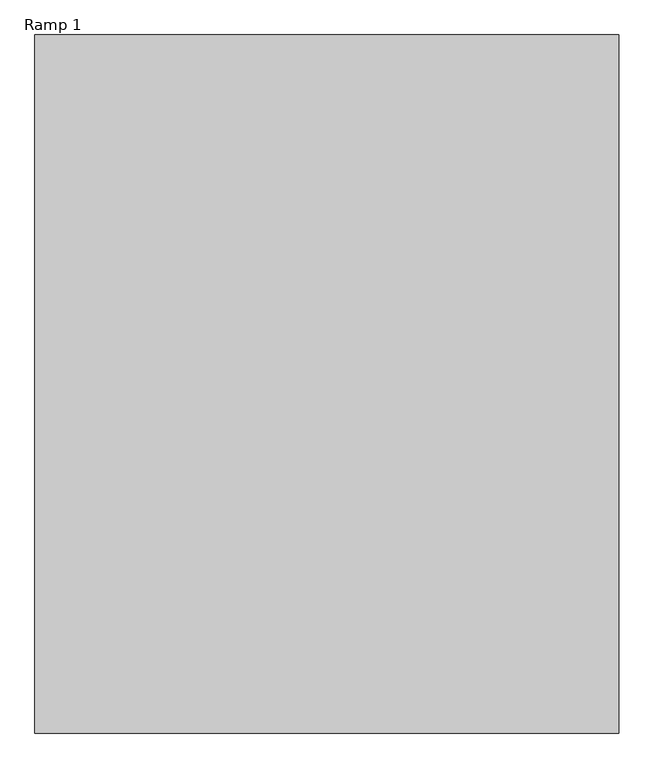
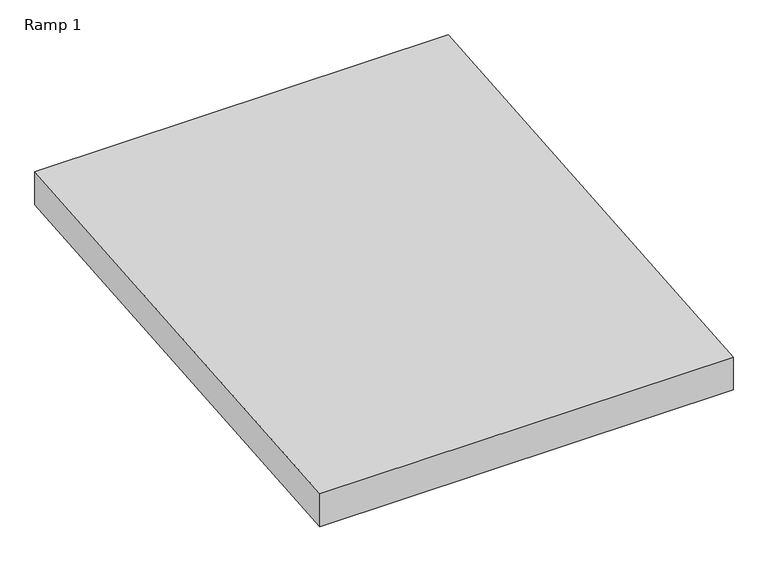
"""IFC4 building model written with IfcOpenShell, lengths in millimetres: ramp geometry, Ramp 1."""

import ifcopenshell
import ifcopenshell.guid

model = None  # the IFC model being written
_history = None  # IfcOwnerHistory: only IFC2X3 demands one
_inside = {}  # id of a spatial element -> (the spatial element, [elements in it])
_under = {}  # id of a project, library or spatial element -> (it, [spatial elements below it])
_declared = {}  # id of a project -> (the project, [libraries it declares])
_typed = {}  # id of a type object -> (the type object, [elements of that type])
_made_of = {}  # id of a material, layer set ... -> (it, [elements and type objects made of it])


def new_model(schema):
    """Start an empty IFC model of exactly this schema.

    Asked for "IFC4X3", IfcOpenShell would pick the latest addendum, in which some entities
    have other attributes; the version numbers below select the first issue.
    IFC2X3 requires an IfcOwnerHistory on every rooted entity: one is made here for all.
    """
    global model, _history
    if schema == "IFC4X3":
        model = ifcopenshell.file(schema_version=(4, 3, 0, 0))
    else:
        model = ifcopenshell.file(schema=schema)
    _inside.clear()
    _under.clear()
    _declared.clear()
    _typed.clear()
    _made_of.clear()
    _history = None
    if model.schema == "IFC2X3":
        org = make("IfcOrganization", Name="unknown")
        user = make(
            "IfcPersonAndOrganization",
            ThePerson=make("IfcPerson", FamilyName="unknown"),
            TheOrganization=org,
        )
        app = make(
            "IfcApplication",
            ApplicationDeveloper=org,
            Version="unknown",
            ApplicationFullName="unknown",
            ApplicationIdentifier="unknown",
        )
        _history = make(
            "IfcOwnerHistory",
            OwningUser=user,
            OwningApplication=app,
            ChangeAction="ADDED",
            CreationDate=0,
        )
    return model


def make(cls, **values):
    """One entity of the class cls with the attributes given. An attribute that is None is left unset."""
    return model.create_entity(
        cls, **{name: value for name, value in values.items() if value is not None}
    )


def rooted(cls, **values):
    """An entity with a GlobalId (a new one), such as an element, a storey or a relation."""
    return make(cls, GlobalId=ifcopenshell.guid.new(), OwnerHistory=_history, **values)


def si_unit(unit_type, name, prefix=None):
    """IfcSIUnit, for example si_unit("LENGTHUNIT", "METRE", prefix="MILLI")."""
    return make("IfcSIUnit", UnitType=unit_type, Prefix=prefix, Name=name)


def assignment(units):
    """IfcUnitAssignment: the units of a project."""
    return None if units is None else make("IfcUnitAssignment", Units=units)


def point(xyz):
    """IfcCartesianPoint."""
    return None if xyz is None else make("IfcCartesianPoint", Coordinates=xyz)


def direction(xyz):
    """IfcDirection."""
    return None if xyz is None else make("IfcDirection", DirectionRatios=xyz)


def frame(location, z_axis=None, x_axis=None):
    """IfcAxis2Placement3D, a coordinate frame: its origin and axes. An axis left out is left unset."""
    return make(
        "IfcAxis2Placement3D",
        Location=point(location),
        Axis=direction(z_axis),
        RefDirection=direction(x_axis),
    )


def origin():
    """The frame at (0, 0, 0) with its axes left unset."""
    return frame((0.0, 0.0, 0.0))


def place(relative_to, where):
    """IfcLocalPlacement: puts the frame where relative to a parent placement (None: the world)."""
    return make(
        "IfcLocalPlacement", PlacementRelTo=relative_to, RelativePlacement=where
    )


def context(
    kind, dimensions, precision=None, world=None, true_north=None, identifier=None
):
    """IfcGeometricRepresentationContext, for example the 3D "Model" context."""
    return make(
        "IfcGeometricRepresentationContext",
        ContextIdentifier=identifier,
        ContextType=kind,
        CoordinateSpaceDimension=dimensions,
        Precision=precision,
        WorldCoordinateSystem=world,
        TrueNorth=true_north,
    )


def project(units=None, contexts=None):
    """IfcProject with its units and contexts."""
    return rooted(
        "IfcProject",
        Name="project",
        RepresentationContexts=contexts,
        UnitsInContext=assignment(units),
    )


def spatial(cls, under=None, at=None, **own):
    """A site, building, storey or space (cls), placed at a placement, below another one or the project."""
    s = rooted(cls, ObjectPlacement=at, **own)
    if under is not None:
        _under.setdefault(under.id(), (under, []))[1].append(s)
    return s


def polyline(points):
    """IfcPolyline through the points."""
    return make("IfcPolyline", Points=[point(p) for p in points])


def outline(outer, holes=None, kind="AREA"):
    """IfcArbitraryClosedProfileDef: a profile drawn as a closed curve; with holes, ...WithVoids."""
    if holes is None:
        return make("IfcArbitraryClosedProfileDef", ProfileType=kind, OuterCurve=outer)
    return make(
        "IfcArbitraryProfileDefWithVoids",
        ProfileType=kind,
        OuterCurve=outer,
        InnerCurves=holes,
    )


def extrude(swept, where, along, depth):
    """IfcExtrudedAreaSolid: the profile swept, set in the frame where, extruded along a direction by depth."""
    return make(
        "IfcExtrudedAreaSolid",
        SweptArea=swept,
        Position=where,
        ExtrudedDirection=direction(along),
        Depth=depth,
    )


def shape(context_of_items, identifier, shape_type, items):
    """IfcShapeRepresentation: the items that make up one representation, for example the "Body"."""
    return make(
        "IfcShapeRepresentation",
        ContextOfItems=context_of_items,
        RepresentationIdentifier=identifier,
        RepresentationType=shape_type,
        Items=items,
    )


def source(mapping_origin, context_of_items, identifier, shape_type, items):
    """IfcRepresentationMap: a shape defined once, which mapped items show again and again."""
    return make(
        "IfcRepresentationMap",
        MappingOrigin=mapping_origin,
        MappedRepresentation=shape(context_of_items, identifier, shape_type, items),
    )


def transform(
    local_origin,
    x_axis=None,
    y_axis=None,
    z_axis=None,
    scale=None,
    scale2=None,
    scale3=None,
    uniform=True,
):
    """IfcCartesianTransformationOperator3D, or its non-uniform kind. x_axis, y_axis, z_axis: its Axis1, 2, 3."""
    if uniform:
        return make(
            "IfcCartesianTransformationOperator3D",
            Axis1=direction(x_axis),
            Axis2=direction(y_axis),
            LocalOrigin=point(local_origin),
            Scale=scale,
            Axis3=direction(z_axis),
        )
    return make(
        "IfcCartesianTransformationOperator3DnonUniform",
        Axis1=direction(x_axis),
        Axis2=direction(y_axis),
        LocalOrigin=point(local_origin),
        Scale=scale,
        Axis3=direction(z_axis),
        Scale2=scale2,
        Scale3=scale3,
    )


def mapped(mapping_source, mapping_target):
    """IfcMappedItem: shows the shape of a source again, moved by a transform."""
    return make(
        "IfcMappedItem", MappingSource=mapping_source, MappingTarget=mapping_target
    )


def made_of(thing, what):
    """Note that an element or type object is made of a material, layer set ...; save() writes the relation."""
    if what is not None:
        _made_of.setdefault(what.id(), (what, []))[1].append(thing)
    return thing


def element(
    cls,
    number,
    at=None,
    inside=None,
    cuts=None,
    type_object=None,
    material=None,
    context=None,
    identifier="Body",
    shape_type=None,
    held_by="IfcProductDefinitionShape",
    body=None,
    shapes=None,
    **own,
):
    """One element of the class cls, such as IfcWall. Its Tag is "e" and its number.

    at: its placement. inside: the storey or other place that contains it. cuts: it is an
    opening in that element (IfcRelVoidsElement). A single representation is given by context,
    identifier, shape_type and body (its items); several are given by shapes. held_by: the class
    of the entity that holds the representations. save() writes the other relations.
    """
    e = rooted(cls, Tag="e%d" % number, ObjectPlacement=at, **own)
    if body is not None:
        shapes = [shape(context, identifier, shape_type, body)]
    if shapes is not None:
        e.Representation = make(held_by, Representations=shapes)
    if inside is not None:
        _inside.setdefault(inside.id(), (inside, []))[1].append(e)
    if cuts is not None:
        rooted(
            "IfcRelVoidsElement", RelatingBuildingElement=cuts, RelatedOpeningElement=e
        )
    if type_object is not None:
        _typed.setdefault(type_object.id(), (type_object, []))[1].append(e)
    return made_of(e, material)


def aggregate(whole, parts):
    """IfcRelAggregates: a whole, such as a stair, and the parts it consists of."""
    return rooted("IfcRelAggregates", RelatingObject=whole, RelatedObjects=parts)


def save(model, path):
    """Write the relations noted so far, then the file.

    IfcRelAggregates (storeys below a building ...), IfcRelContainedInSpatialStructure (elements
    in a storey), IfcRelDefinesByType, IfcRelAssociatesMaterial and IfcRelDeclares: one each for
    every whole, place, type object, material and project.
    """
    for whole, parts in _under.values():
        aggregate(whole, parts)
    for where, things in _inside.values():
        rooted(
            "IfcRelContainedInSpatialStructure",
            RelatedElements=things,
            RelatingStructure=where,
        )
    for kind, things in _typed.values():
        rooted("IfcRelDefinesByType", RelatedObjects=things, RelatingType=kind)
    for what, things in _made_of.values():
        rooted("IfcRelAssociatesMaterial", RelatedObjects=things, RelatingMaterial=what)
    for by, libraries in _declared.values():
        rooted("IfcRelDeclares", RelatingContext=by, RelatedDefinitions=libraries)
    model.write(path)


def ramp_1_1c041b4d(model_context):
    return source(origin(), model_context, "Body", "SweptSolid", [
        extrude(outline(polyline([(-588.7354398, 0.0), (1550.939444, 178.3062403), (1550.939444, 27.7863081), (-588.7354398, -150.5199322), (-588.7354398, 0.0)])), frame((5737.3508412, 0.0, 0.0), z_axis=(1.0, 0.0, 0.0), x_axis=(0.0, 1.0, 0.0)), (0.0, 0.0, 1.0), 1790.0),
    ])


if __name__ == "__main__":
    model = new_model("IFC4")
    model_context = context("Model", 3, world=origin())
    ifc_project = project(units=[si_unit("LENGTHUNIT", "METRE", prefix="MILLI")], contexts=[model_context])
    site = spatial("IfcSite", under=ifc_project)
    building = spatial("IfcBuilding", under=site)
    placement = place(None, origin())
    ramp_1_shape = ramp_1_1c041b4d(model_context)
    element("IfcRamp", 1, ObjectType="Ramp 1", at=placement, inside=building, context=model_context, shape_type="MappedRepresentation", body=[
        mapped(ramp_1_shape, transform((0.0, 0.0, 0.0), x_axis=(1.0, 0.0, 0.0), y_axis=(0.0, 1.0, 0.0), z_axis=(0.0, 0.0, 1.0))),
    ])
    save(model, "model.ifc")
